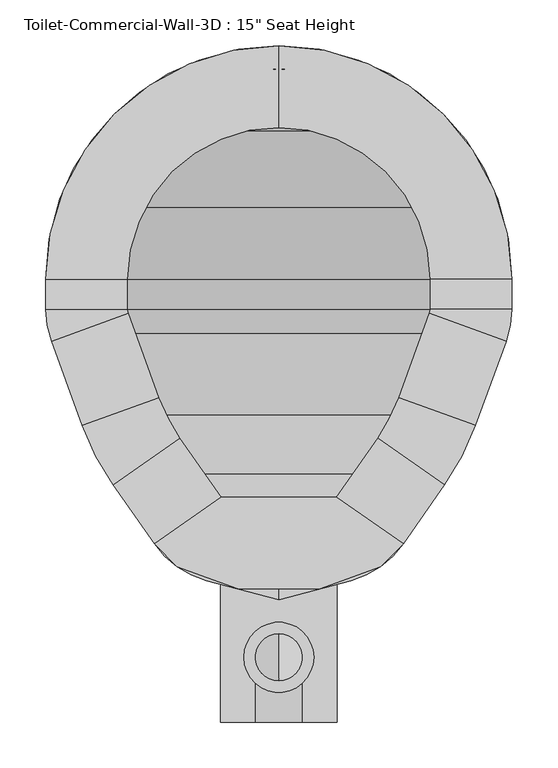
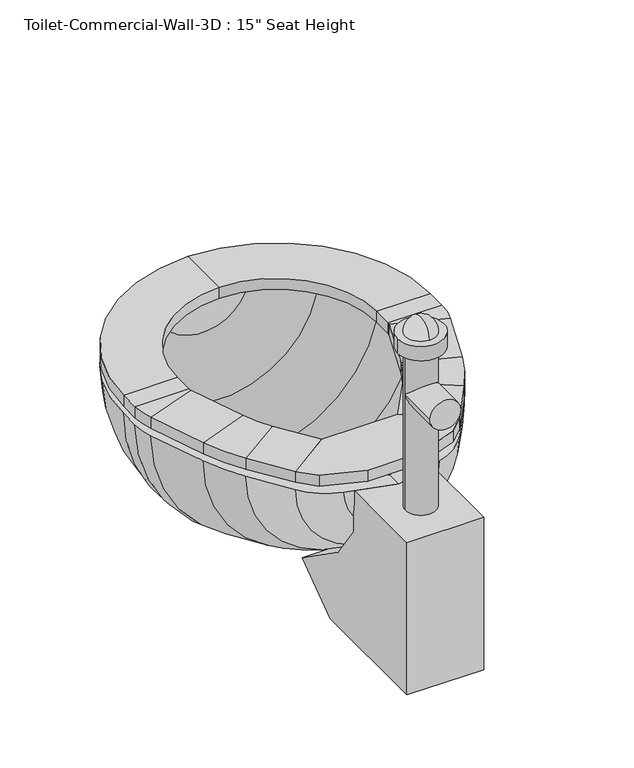
"""IFC4 building model written with IfcOpenShell, lengths in millimetres: flow terminal geometry."""

import ifcopenshell
import ifcopenshell.guid

model = None  # the IFC model being written
_history = None  # IfcOwnerHistory: only IFC2X3 demands one
_inside = {}  # id of a spatial element -> (the spatial element, [elements in it])
_under = {}  # id of a project, library or spatial element -> (it, [spatial elements below it])
_declared = {}  # id of a project -> (the project, [libraries it declares])
_typed = {}  # id of a type object -> (the type object, [elements of that type])
_made_of = {}  # id of a material, layer set ... -> (it, [elements and type objects made of it])


def new_model(schema):
    """Start an empty IFC model of exactly this schema.

    Asked for "IFC4X3", IfcOpenShell would pick the latest addendum, in which some entities
    have other attributes; the version numbers below select the first issue.
    IFC2X3 requires an IfcOwnerHistory on every rooted entity: one is made here for all.
    """
    global model, _history
    if schema == "IFC4X3":
        model = ifcopenshell.file(schema_version=(4, 3, 0, 0))
    else:
        model = ifcopenshell.file(schema=schema)
    _inside.clear()
    _under.clear()
    _declared.clear()
    _typed.clear()
    _made_of.clear()
    _history = None
    if model.schema == "IFC2X3":
        org = make("IfcOrganization", Name="unknown")
        user = make(
            "IfcPersonAndOrganization",
            ThePerson=make("IfcPerson", FamilyName="unknown"),
            TheOrganization=org,
        )
        app = make(
            "IfcApplication",
            ApplicationDeveloper=org,
            Version="unknown",
            ApplicationFullName="unknown",
            ApplicationIdentifier="unknown",
        )
        _history = make(
            "IfcOwnerHistory",
            OwningUser=user,
            OwningApplication=app,
            ChangeAction="ADDED",
            CreationDate=0,
        )
    return model


def make(cls, **values):
    """One entity of the class cls with the attributes given. An attribute that is None is left unset."""
    return model.create_entity(
        cls, **{name: value for name, value in values.items() if value is not None}
    )


def rooted(cls, **values):
    """An entity with a GlobalId (a new one), such as an element, a storey or a relation."""
    return make(cls, GlobalId=ifcopenshell.guid.new(), OwnerHistory=_history, **values)


def si_unit(unit_type, name, prefix=None):
    """IfcSIUnit, for example si_unit("LENGTHUNIT", "METRE", prefix="MILLI")."""
    return make("IfcSIUnit", UnitType=unit_type, Prefix=prefix, Name=name)


def assignment(units):
    """IfcUnitAssignment: the units of a project."""
    return None if units is None else make("IfcUnitAssignment", Units=units)


def point(xyz):
    """IfcCartesianPoint."""
    return None if xyz is None else make("IfcCartesianPoint", Coordinates=xyz)


def direction(xyz):
    """IfcDirection."""
    return None if xyz is None else make("IfcDirection", DirectionRatios=xyz)


def frame(location, z_axis=None, x_axis=None):
    """IfcAxis2Placement3D, a coordinate frame: its origin and axes. An axis left out is left unset."""
    return make(
        "IfcAxis2Placement3D",
        Location=point(location),
        Axis=direction(z_axis),
        RefDirection=direction(x_axis),
    )


def frame_2d(location, x_axis=None):
    """IfcAxis2Placement2D, a coordinate frame in the plane: its origin and x axis."""
    return make(
        "IfcAxis2Placement2D", Location=point(location), RefDirection=direction(x_axis)
    )


def origin():
    """The frame at (0, 0, 0) with its axes left unset."""
    return frame((0.0, 0.0, 0.0))


def place(relative_to, where):
    """IfcLocalPlacement: puts the frame where relative to a parent placement (None: the world)."""
    return make(
        "IfcLocalPlacement", PlacementRelTo=relative_to, RelativePlacement=where
    )


def context(
    kind, dimensions, precision=None, world=None, true_north=None, identifier=None
):
    """IfcGeometricRepresentationContext, for example the 3D "Model" context."""
    return make(
        "IfcGeometricRepresentationContext",
        ContextIdentifier=identifier,
        ContextType=kind,
        CoordinateSpaceDimension=dimensions,
        Precision=precision,
        WorldCoordinateSystem=world,
        TrueNorth=true_north,
    )


def project(units=None, contexts=None):
    """IfcProject with its units and contexts."""
    return rooted(
        "IfcProject",
        Name="project",
        RepresentationContexts=contexts,
        UnitsInContext=assignment(units),
    )


def spatial(cls, under=None, at=None, **own):
    """A site, building, storey or space (cls), placed at a placement, below another one or the project."""
    s = rooted(cls, ObjectPlacement=at, **own)
    if under is not None:
        _under.setdefault(under.id(), (under, []))[1].append(s)
    return s


def polyline(points):
    """IfcPolyline through the points."""
    return make("IfcPolyline", Points=[point(p) for p in points])


def circle_curve(where, radius):
    """IfcCircle in the frame where."""
    return make("IfcCircle", Position=where, Radius=radius)


def ellipse_curve(where, semi_axis1, semi_axis2):
    """IfcEllipse in the frame where."""
    return make(
        "IfcEllipse", Position=where, SemiAxis1=semi_axis1, SemiAxis2=semi_axis2
    )


def trimmed(basis, trim1, trim2, sense, master):
    """IfcTrimmedCurve: the piece of a basis curve between two trims."""
    return make(
        "IfcTrimmedCurve",
        BasisCurve=basis,
        Trim1=trim1,
        Trim2=trim2,
        SenseAgreement=sense,
        MasterRepresentation=master,
    )


def segment(curve, same_sense, transition):
    """IfcCompositeCurveSegment."""
    return make(
        "IfcCompositeCurveSegment",
        Transition=transition,
        SameSense=same_sense,
        ParentCurve=curve,
    )


def composite_curve(segments, self_intersect=None):
    """IfcCompositeCurve: segments joined end to end."""
    return make("IfcCompositeCurve", Segments=segments, SelfIntersect=self_intersect)


def outline(outer, holes=None, kind="AREA"):
    """IfcArbitraryClosedProfileDef: a profile drawn as a closed curve; with holes, ...WithVoids."""
    if holes is None:
        return make("IfcArbitraryClosedProfileDef", ProfileType=kind, OuterCurve=outer)
    return make(
        "IfcArbitraryProfileDefWithVoids",
        ProfileType=kind,
        OuterCurve=outer,
        InnerCurves=holes,
    )


def extrude(swept, where, along, depth):
    """IfcExtrudedAreaSolid: the profile swept, set in the frame where, extruded along a direction by depth."""
    return make(
        "IfcExtrudedAreaSolid",
        SweptArea=swept,
        Position=where,
        ExtrudedDirection=direction(along),
        Depth=depth,
    )


def shape(context_of_items, identifier, shape_type, items):
    """IfcShapeRepresentation: the items that make up one representation, for example the "Body"."""
    return make(
        "IfcShapeRepresentation",
        ContextOfItems=context_of_items,
        RepresentationIdentifier=identifier,
        RepresentationType=shape_type,
        Items=items,
    )


def source(mapping_origin, context_of_items, identifier, shape_type, items):
    """IfcRepresentationMap: a shape defined once, which mapped items show again and again."""
    return make(
        "IfcRepresentationMap",
        MappingOrigin=mapping_origin,
        MappedRepresentation=shape(context_of_items, identifier, shape_type, items),
    )


def transform(
    local_origin,
    x_axis=None,
    y_axis=None,
    z_axis=None,
    scale=None,
    scale2=None,
    scale3=None,
    uniform=True,
):
    """IfcCartesianTransformationOperator3D, or its non-uniform kind. x_axis, y_axis, z_axis: its Axis1, 2, 3."""
    if uniform:
        return make(
            "IfcCartesianTransformationOperator3D",
            Axis1=direction(x_axis),
            Axis2=direction(y_axis),
            LocalOrigin=point(local_origin),
            Scale=scale,
            Axis3=direction(z_axis),
        )
    return make(
        "IfcCartesianTransformationOperator3DnonUniform",
        Axis1=direction(x_axis),
        Axis2=direction(y_axis),
        LocalOrigin=point(local_origin),
        Scale=scale,
        Axis3=direction(z_axis),
        Scale2=scale2,
        Scale3=scale3,
    )


def mapped(mapping_source, mapping_target):
    """IfcMappedItem: shows the shape of a source again, moved by a transform."""
    return make(
        "IfcMappedItem", MappingSource=mapping_source, MappingTarget=mapping_target
    )


def made_of(thing, what):
    """Note that an element or type object is made of a material, layer set ...; save() writes the relation."""
    if what is not None:
        _made_of.setdefault(what.id(), (what, []))[1].append(thing)
    return thing


def element(
    cls,
    number,
    at=None,
    inside=None,
    cuts=None,
    type_object=None,
    material=None,
    context=None,
    identifier="Body",
    shape_type=None,
    held_by="IfcProductDefinitionShape",
    body=None,
    shapes=None,
    **own,
):
    """One element of the class cls, such as IfcWall. Its Tag is "e" and its number.

    at: its placement. inside: the storey or other place that contains it. cuts: it is an
    opening in that element (IfcRelVoidsElement). A single representation is given by context,
    identifier, shape_type and body (its items); several are given by shapes. held_by: the class
    of the entity that holds the representations. save() writes the other relations.
    """
    e = rooted(cls, Tag="e%d" % number, ObjectPlacement=at, **own)
    if body is not None:
        shapes = [shape(context, identifier, shape_type, body)]
    if shapes is not None:
        e.Representation = make(held_by, Representations=shapes)
    if inside is not None:
        _inside.setdefault(inside.id(), (inside, []))[1].append(e)
    if cuts is not None:
        rooted(
            "IfcRelVoidsElement", RelatingBuildingElement=cuts, RelatedOpeningElement=e
        )
    if type_object is not None:
        _typed.setdefault(type_object.id(), (type_object, []))[1].append(e)
    return made_of(e, material)


def aggregate(whole, parts):
    """IfcRelAggregates: a whole, such as a stair, and the parts it consists of."""
    return rooted("IfcRelAggregates", RelatingObject=whole, RelatedObjects=parts)


def save(model, path):
    """Write the relations noted so far, then the file.

    IfcRelAggregates (storeys below a building ...), IfcRelContainedInSpatialStructure (elements
    in a storey), IfcRelDefinesByType, IfcRelAssociatesMaterial and IfcRelDeclares: one each for
    every whole, place, type object, material and project.
    """
    for whole, parts in _under.values():
        aggregate(whole, parts)
    for where, things in _inside.values():
        rooted(
            "IfcRelContainedInSpatialStructure",
            RelatedElements=things,
            RelatingStructure=where,
        )
    for kind, things in _typed.values():
        rooted("IfcRelDefinesByType", RelatedObjects=things, RelatingType=kind)
    for what, things in _made_of.values():
        rooted("IfcRelAssociatesMaterial", RelatedObjects=things, RelatingMaterial=what)
    for by, libraries in _declared.values():
        rooted("IfcRelDeclares", RelatingContext=by, RelatedDefinitions=libraries)
    model.write(path)


def plane_surface(at):
    """IfcPlane: the flat surface through the origin of the frame at, square to its z axis."""
    return make("IfcPlane", Position=at)


def cylinder_surface(at, radius):
    """IfcCylindricalSurface: all points at the distance radius from the z axis of the frame at."""
    return make("IfcCylindricalSurface", Position=at, Radius=radius)


def revolved_surface(curve, axis_point, axis_direction):
    """IfcSurfaceOfRevolution: the curve turned about the line through axis_point along axis_direction."""
    return make(
        "IfcSurfaceOfRevolution",
        SweptCurve=make("IfcArbitraryOpenProfileDef", ProfileType="CURVE", Curve=curve),
        AxisPosition=make("IfcAxis1Placement", Location=point(axis_point), Axis=direction(axis_direction)),
    )


def advanced_brep(points, edges, surfaces, faces):
    """IfcAdvancedBrep: a solid bounded by faces that lie on surfaces and meet in shared edges.

    An edge is (start, end): straight between two places in points (the first is 0);
    or (start, end, curve); or (start, end, curve, False) where it runs against its curve.
    A face is (place in surfaces, loops), or (place, loops, False) where it looks against
    its surface's normal. A loop lists edges by number (the first is 1), with a minus sign
    where the edge is run from its end to its start. The first loop is the outer one.
    """
    corners = [point(p) for p in points]
    vertices = [make("IfcVertexPoint", VertexGeometry=c) for c in corners]
    made = []
    for start, end, *more in edges:
        made.append(
            make(
                "IfcEdgeCurve",
                EdgeStart=vertices[start],
                EdgeEnd=vertices[end],
                EdgeGeometry=more[0] if more else make("IfcPolyline", Points=[corners[start], corners[end]]),
                SameSense=more[1] if len(more) > 1 else True,
            )
        )
    hull = []
    for where, loops, *sense in faces:
        bounds = []
        for j, loop in enumerate(loops):
            ring = [make("IfcOrientedEdge", EdgeElement=made[abs(k) - 1], Orientation=k > 0) for k in loop]
            bounds.append(
                make(
                    "IfcFaceOuterBound" if j == 0 else "IfcFaceBound",
                    Bound=make("IfcEdgeLoop", EdgeList=ring),
                    Orientation=True,
                )
            )
        hull.append(make("IfcAdvancedFace", Bounds=bounds, FaceSurface=surfaces[where], SameSense=sense[0] if sense else True))
    return make("IfcAdvancedBrep", Outer=make("IfcClosedShell", CfsFaces=hull))


def flow_terminal_fb6ce90a(model_context):
    return source(origin(), model_context, "Body", "SolidModel", [
        extrude(outline(polyline([(467.7541169, 443.4722495), (540.5767337, 392.4813043), (515.6262519, 367.5308226), (449.563909, 343.4860961), (360.2423986, 343.4860961), (294.1800557, 367.5308226), (269.229574, 392.4813043), (342.0521907, 443.4722495), (467.7541169, 443.4722495)])), frame((0.0, 0.0, 355.6), z_axis=(0.0, 0.0, 1.0), x_axis=(1.0, 0.0, 0.0)), (0.0, 0.0, 1.0), 19.05),
        advanced_brep(
        [(467.7541169, 443.4722495, 355.6), (540.5767337, 392.4813043, 355.6), (540.5767337, 392.4813043, 374.65), (467.7541169, 443.4722495, 374.65), (512.8583992, 507.8878403, 355.6), (585.6810159, 456.8968951, 355.6), (585.6810159, 456.8968951, 374.65), (512.8583992, 507.8878403, 374.65), (619.360053, 521.5937234, 355.6), (535.821379, 551.9993141, 355.6), (619.360053, 521.5937234, 374.65), (535.821379, 551.9993141, 374.65), (569.2372501, 643.8086654, 355.6), (652.7759241, 613.4030747, 355.6), (652.7759241, 613.4030747, 374.65), (569.2372501, 643.8086654, 374.65), (658.9031538, 648.1523212, 355.6), (570.0031538, 648.1523212, 355.6), (658.9031538, 648.1523212, 374.65), (570.0031538, 648.1523212, 374.65), (570.0031538, 681.0375, 355.6), (658.9031538, 681.0375, 355.6), (658.9031538, 681.0375, 374.65), (570.0031538, 681.0375, 374.65), (404.9031538, 935.0375, 355.6), (404.9031538, 846.1375, 355.6), (404.9031538, 935.0375, 374.65), (404.9031538, 846.1375, 374.65), (150.9031538, 681.0375, 355.6), (239.8031538, 681.0375, 355.6), (150.9031538, 681.0375, 374.65), (239.8031538, 681.0375, 374.65), (239.8031538, 648.1523212, 355.6), (150.9031538, 648.1523212, 355.6), (150.9031538, 648.1523212, 374.65), (239.8031538, 648.1523212, 374.65), (157.0303835, 613.4030747, 355.6), (240.5690575, 643.8086654, 355.6), (157.0303835, 613.4030747, 374.65), (240.5690575, 643.8086654, 374.65), (273.9849286, 551.9993141, 355.6), (190.4462546, 521.5937234, 355.6), (190.4462546, 521.5937234, 374.65), (273.9849286, 551.9993141, 374.65), (224.1252917, 456.8968951, 355.6), (296.9479084, 507.8878403, 355.6), (224.1252917, 456.8968951, 374.65), (296.9479084, 507.8878403, 374.65), (342.0521907, 443.4722495, 355.6), (342.0521907, 443.4722495, 374.65), (269.229574, 392.4813043, 374.65), (269.229574, 392.4813043, 355.6)],
        [
            (0, 1),
            (1, 2),
            (2, 3),
            (3, 0),
            (0, 4),
            (4, 5),
            (5, 1),
            (5, 6),
            (6, 2),
            (6, 7),
            (7, 3),
            (7, 4),
            (8, 5, circle_curve(frame((356.8099347, 617.1541514, 355.6), z_axis=(0.0, 0.0, -1.0), x_axis=(0.81915204428899, -0.5735764363510486, 0.0)), 279.4)),
            (4, 9, circle_curve(frame((356.8099347, 617.1541514, 355.6), z_axis=(0.0, 0.0, 1.0), x_axis=(0.81915204428899, -0.5735764363510486, 0.0)), 190.5)),
            (9, 8),
            (10, 6, circle_curve(frame((356.8099347, 617.1541514, 374.65), z_axis=(0.0, 0.0, -1.0), x_axis=(0.81915204428899, -0.5735764363510486, 0.0)), 279.4)),
            (8, 10),
            (11, 7, circle_curve(frame((356.8099347, 617.1541514, 374.65), z_axis=(0.0, 0.0, -1.0), x_axis=(0.81915204428899, -0.5735764363510486, 0.0)), 190.5)),
            (10, 11),
            (11, 9),
            (9, 12),
            (12, 13),
            (13, 8),
            (13, 14),
            (14, 10),
            (14, 15),
            (15, 11),
            (15, 12),
            (16, 13, circle_curve(frame((557.3031538, 648.1523212, 355.6), z_axis=(0.0, 0.0, -1.0), x_axis=(0.9396926207859057, -0.3420201433256761, 0.0)), 101.6)),
            (12, 17, circle_curve(frame((557.3031538, 648.1523212, 355.6), z_axis=(0.0, 0.0, 1.0), x_axis=(0.9396926207859057, -0.3420201433256761, 0.0)), 12.7)),
            (17, 16),
            (18, 14, circle_curve(frame((557.3031538, 648.1523212, 374.65), z_axis=(0.0, 0.0, -1.0), x_axis=(0.9396926207859057, -0.3420201433256761, 0.0)), 101.6)),
            (16, 18),
            (19, 15, circle_curve(frame((557.3031538, 648.1523212, 374.65), z_axis=(0.0, 0.0, -1.0), x_axis=(0.9396926207859057, -0.3420201433256761, 0.0)), 12.7)),
            (18, 19),
            (19, 17),
            (17, 20),
            (20, 21),
            (21, 16),
            (21, 22),
            (22, 18),
            (22, 23),
            (23, 19),
            (23, 20),
            (24, 21, circle_curve(frame((404.9031538, 681.0375, 355.6), z_axis=(0.0, 0.0, -1.0), x_axis=(1.0, 0.0, 0.0)), 254.0)),
            (20, 25, circle_curve(frame((404.9031538, 681.0375, 355.6), z_axis=(0.0, 0.0, 1.0), x_axis=(1.0, 0.0, 0.0)), 165.1)),
            (25, 24),
            (26, 22, circle_curve(frame((404.9031538, 681.0375, 374.65), z_axis=(0.0, 0.0, -1.0), x_axis=(1.0, 0.0, 0.0)), 254.0)),
            (24, 26),
            (27, 23, circle_curve(frame((404.9031538, 681.0375, 374.65), z_axis=(0.0, 0.0, -1.0), x_axis=(1.0, 0.0, 0.0)), 165.1)),
            (26, 27),
            (27, 25),
            (28, 24, circle_curve(frame((404.9031538, 681.0375, 355.6), z_axis=(0.0, 0.0, -1.0), x_axis=(0.0, 1.0, 0.0)), 254.0)),
            (25, 29, circle_curve(frame((404.9031538, 681.0375, 355.6), z_axis=(0.0, 0.0, 1.0), x_axis=(0.0, 1.0, 0.0)), 165.1)),
            (29, 28),
            (30, 26, circle_curve(frame((404.9031538, 681.0375, 374.65), z_axis=(0.0, 0.0, -1.0), x_axis=(0.0, 1.0, 0.0)), 254.0)),
            (28, 30),
            (31, 27, circle_curve(frame((404.9031538, 681.0375, 374.65), z_axis=(0.0, 0.0, -1.0), x_axis=(0.0, 1.0, 0.0)), 165.1)),
            (30, 31),
            (31, 29),
            (29, 32),
            (32, 33),
            (33, 28),
            (33, 34),
            (34, 30),
            (34, 35),
            (35, 31),
            (35, 32),
            (36, 33, circle_curve(frame((252.5031538, 648.1523212, 355.6), z_axis=(0.0, 0.0, -1.0), x_axis=(-1.0, 0.0, 0.0)), 101.6)),
            (32, 37, circle_curve(frame((252.5031538, 648.1523212, 355.6), z_axis=(0.0, 0.0, 1.0), x_axis=(-1.0, 0.0, 0.0)), 12.7)),
            (37, 36),
            (38, 34, circle_curve(frame((252.5031538, 648.1523212, 374.65), z_axis=(0.0, 0.0, -1.0), x_axis=(-1.0, 0.0, 0.0)), 101.6)),
            (36, 38),
            (39, 35, circle_curve(frame((252.5031538, 648.1523212, 374.65), z_axis=(0.0, 0.0, -1.0), x_axis=(-1.0, 0.0, 0.0)), 12.7)),
            (38, 39),
            (39, 37),
            (37, 40),
            (40, 41),
            (41, 36),
            (41, 42),
            (42, 38),
            (42, 43),
            (43, 39),
            (43, 40),
            (44, 41, circle_curve(frame((452.9963729, 617.1541514, 355.6), z_axis=(0.0, 0.0, -1.0), x_axis=(-0.939692620785909, -0.3420201433256672, 0.0)), 279.4)),
            (40, 45, circle_curve(frame((452.9963729, 617.1541514, 355.6), z_axis=(0.0, 0.0, 1.0), x_axis=(-0.939692620785909, -0.3420201433256672, 0.0)), 190.5)),
            (45, 44),
            (46, 42, circle_curve(frame((452.9963729, 617.1541514, 374.65), z_axis=(0.0, 0.0, -1.0), x_axis=(-0.939692620785909, -0.3420201433256672, 0.0)), 279.4)),
            (44, 46),
            (47, 43, circle_curve(frame((452.9963729, 617.1541514, 374.65), z_axis=(0.0, 0.0, -1.0), x_axis=(-0.939692620785909, -0.3420201433256672, 0.0)), 190.5)),
            (46, 47),
            (47, 45),
            (48, 49),
            (49, 50),
            (50, 51),
            (51, 48),
            (45, 48),
            (51, 44),
            (50, 46),
            (49, 47),
        ],
        [
            plane_surface(frame((540.5767337, 392.4813043, 437.2995365), z_axis=(-0.5735764363510436, -0.8191520442889937, 0.0), x_axis=(0.8191520442889937, -0.5735764363510436, 0.0))),
            plane_surface(frame((467.7541169, 443.4722495, 355.6), z_axis=(0.0, 0.0, -1.0), x_axis=(0.5735764363510436, 0.8191520442889936, 0.0))),
            plane_surface(frame((540.5767337, 392.4813043, 355.6), z_axis=(0.8191520442889944, -0.5735764363510424, 0.0), x_axis=(0.5735764363510424, 0.8191520442889944, 0.0))),
            plane_surface(frame((540.5767337, 392.4813043, 374.65), z_axis=(0.0, 0.0, 1.0), x_axis=(0.573576436351043, 0.819152044288994, 0.0))),
            plane_surface(frame((467.7541169, 443.4722495, 374.65), z_axis=(-0.819152044288994, 0.573576436351043, 0.0), x_axis=(0.573576436351043, 0.819152044288994, 0.0))),
            plane_surface(frame((356.8099347, 617.1541514, 355.6), z_axis=(0.0, 0.0, -1.0), x_axis=(0.81915204428899, -0.5735764363510486, 0.0))),
            cylinder_surface(frame((356.8099347, 617.1541514, 342.9), z_axis=(0.0, 0.0, 1.0), x_axis=(0.81915204428899, -0.5735764363510486, 0.0)), 279.4),
            plane_surface(frame((356.8099347, 617.1541514, 374.65), z_axis=(0.0, 0.0, 1.0), x_axis=(0.81915204428899, -0.5735764363510486, 0.0))),
            revolved_surface(polyline([(512.8583991370526, 507.8878402751253, 374.65), (512.8583991370526, 507.8878402751253, 355.6)]), (356.8099347, 617.1541514, 342.9), (0.0, 0.0, 1.0)),
            plane_surface(frame((535.821379, 551.9993141, 355.6), z_axis=(0.0, 0.0, -1.0000000000000002), x_axis=(0.3420201433256594, 0.9396926207859119, 0.0))),
            plane_surface(frame((619.360053, 521.5937234, 355.6), z_axis=(0.9396926207859121, -0.3420201433256587, 0.0), x_axis=(0.3420201433256587, 0.9396926207859121, 0.0))),
            plane_surface(frame((619.360053, 521.5937234, 374.65), z_axis=(0.0, 0.0, 1.0), x_axis=(0.34202014332565916, 0.9396926207859119, 0.0))),
            plane_surface(frame((535.821379, 551.9993141, 374.65), z_axis=(-0.9396926207859122, 0.34202014332565833, 0.0), x_axis=(0.34202014332565833, 0.9396926207859122, 0.0))),
            plane_surface(frame((557.3031538, 648.1523212, 355.6), z_axis=(0.0, 0.0, -1.0000000000000002), x_axis=(0.9396926207859058, -0.34202014332567615, 0.0))),
            cylinder_surface(frame((557.3031538, 648.1523212, 342.9), z_axis=(0.0, 0.0, 1.0), x_axis=(0.9396926207859057, -0.3420201433256761, 0.0)), 101.6),
            plane_surface(frame((557.3031538, 648.1523212, 374.65), z_axis=(0.0, 0.0, 1.0000000000000002), x_axis=(0.9396926207859058, -0.34202014332567615, 0.0))),
            revolved_surface(polyline([(569.237250083981, 643.8086653797639, 374.65), (569.237250083981, 643.8086653797639, 355.6)]), (557.3031538, 648.1523212, 342.9), (0.0, 0.0, 1.0)),
            plane_surface(frame((570.0031538, 648.1523212, 355.6), z_axis=(0.0, 0.0, -1.0), x_axis=(0.0, 1.0, 0.0))),
            plane_surface(frame((658.9031538, 648.1523212, 355.6), z_axis=(1.0, 0.0, 0.0), x_axis=(0.0, 1.0, 0.0))),
            plane_surface(frame((658.9031538, 648.1523212, 374.65), z_axis=(0.0, 0.0, 1.0), x_axis=(0.0, 1.0, 0.0))),
            plane_surface(frame((570.0031538, 648.1523212, 374.65), z_axis=(-1.0, 0.0, 0.0), x_axis=(0.0, 1.0, 0.0))),
            plane_surface(frame((404.9031538, 681.0375, 355.6), z_axis=(0.0, 0.0, -1.0), x_axis=(1.0, 0.0, 0.0))),
            cylinder_surface(frame((404.9031538, 681.0375, 342.9), z_axis=(0.0, 0.0, 1.0), x_axis=(1.0, 0.0, 0.0)), 254.0),
            plane_surface(frame((404.9031538, 681.0375, 374.65), z_axis=(0.0, 0.0, 1.0), x_axis=(1.0, 0.0, 0.0))),
            revolved_surface(polyline([(570.0031538, 681.0375, 374.65), (570.0031538, 681.0375, 355.6)]), (404.9031538, 681.0375, 342.9), (0.0, 0.0, 1.0)),
            plane_surface(frame((404.9031538, 681.0375, 355.6), z_axis=(0.0, 0.0, -1.0), x_axis=(0.0, 1.0, 0.0))),
            cylinder_surface(frame((404.9031538, 681.0375, 342.9), z_axis=(0.0, 0.0, 1.0), x_axis=(0.0, 1.0, 0.0)), 254.0),
            plane_surface(frame((404.9031538, 681.0375, 374.65), z_axis=(0.0, 0.0, 1.0), x_axis=(0.0, 1.0, 0.0))),
            revolved_surface(polyline([(404.9031538, 846.1375, 374.65), (404.9031538, 846.1375, 355.6)]), (404.9031538, 681.0375, 342.9), (0.0, 0.0, 1.0)),
            plane_surface(frame((239.8031538, 681.0375, 355.6), z_axis=(0.0, 0.0, -1.0), x_axis=(0.0, -1.0, 0.0))),
            plane_surface(frame((150.9031538, 681.0375, 355.6), z_axis=(-1.0, 0.0, 0.0), x_axis=(0.0, -1.0, 0.0))),
            plane_surface(frame((150.9031538, 681.0375, 374.65), z_axis=(0.0, 0.0, 1.0), x_axis=(0.0, -1.0, 0.0))),
            plane_surface(frame((239.8031538, 681.0375, 374.65), z_axis=(1.0, 0.0, 0.0), x_axis=(0.0, -1.0, 0.0))),
            plane_surface(frame((252.5031538, 648.1523212, 355.6), z_axis=(0.0, 0.0, -1.0), x_axis=(-1.0, 0.0, 0.0))),
            cylinder_surface(frame((252.5031538, 648.1523212, 342.9), z_axis=(0.0, 0.0, 1.0), x_axis=(-1.0, 0.0, 0.0)), 101.6),
            plane_surface(frame((252.5031538, 648.1523212, 374.65), z_axis=(0.0, 0.0, 1.0), x_axis=(-1.0, 0.0, 0.0))),
            revolved_surface(polyline([(239.80315380000002, 648.1523212, 374.65), (239.80315380000002, 648.1523212, 355.6)]), (252.5031538, 648.1523212, 342.9), (0.0, 0.0, 1.0)),
            plane_surface(frame((240.5690575, 643.8086654, 355.6), z_axis=(0.0, 0.0, -1.0), x_axis=(0.3420201433256581, -0.9396926207859123, 0.0))),
            plane_surface(frame((157.0303835, 613.4030747, 355.6), z_axis=(-0.9396926207859122, -0.3420201433256583, 0.0), x_axis=(0.3420201433256583, -0.9396926207859122, 0.0))),
            plane_surface(frame((157.0303835, 613.4030747, 374.65), z_axis=(0.0, 0.0, 1.0), x_axis=(0.34202014332565855, -0.9396926207859121, 0.0))),
            plane_surface(frame((240.5690575, 643.8086654, 374.65), z_axis=(0.9396926207859124, 0.3420201433256579, 0.0), x_axis=(0.3420201433256579, -0.9396926207859124, 0.0))),
            plane_surface(frame((452.9963729, 617.1541514, 355.6), z_axis=(0.0, 0.0, -1.0), x_axis=(-0.939692620785909, -0.3420201433256672, 0.0))),
            cylinder_surface(frame((452.9963729, 617.1541514, 342.9), z_axis=(0.0, 0.0, 1.0), x_axis=(-0.939692620785909, -0.3420201433256672, 0.0)), 279.4),
            plane_surface(frame((452.9963729, 617.1541514, 374.65), z_axis=(0.0, 0.0, 1.0), x_axis=(-0.939692620785909, -0.3420201433256672, 0.0))),
            revolved_surface(polyline([(273.98492864028435, 551.9993140964605, 374.65), (273.98492864028435, 551.9993140964605, 355.6)]), (452.9963729, 617.1541514, 342.9), (0.0, 0.0, 1.0)),
            plane_surface(frame((269.229574, 392.4813043, 248.5004635), z_axis=(0.5735764363510469, -0.8191520442889914, 0.0), x_axis=(0.8191520442889914, 0.5735764363510469, 0.0))),
            plane_surface(frame((296.9479084, 507.8878403, 355.6), z_axis=(0.0, 0.0, -1.0), x_axis=(0.5735764363510465, -0.8191520442889916, 0.0))),
            plane_surface(frame((224.1252917, 456.8968951, 355.6), z_axis=(-0.819152044288991, -0.5735764363510473, 0.0), x_axis=(0.5735764363510473, -0.819152044288991, 0.0))),
            plane_surface(frame((224.1252917, 456.8968951, 374.65), z_axis=(0.0, 0.0, 1.0), x_axis=(0.5735764363510473, -0.819152044288991, 0.0))),
            plane_surface(frame((296.9479084, 507.8878403, 374.65), z_axis=(0.8191520442889914, 0.5735764363510468, 0.0), x_axis=(0.5735764363510468, -0.8191520442889914, 0.0))),
        ],
        [
            (0, [[1, 2, 3, 4]]),
            (1, [[-1, 5, 6, 7]]),
            (2, [[-2, -7, 8, 9]]),
            (3, [[-3, -9, 10, 11]]),
            (4, [[-4, -11, 12, -5]]),
            (5, [[13, -6, 14, 15]]),
            (6, [[16, -8, -13, 17]]),
            (7, [[18, -10, -16, 19]]),
            (8, [[-14, -12, -18, 20]]),
            (9, [[-15, 21, 22, 23]]),
            (10, [[-17, -23, 24, 25]]),
            (11, [[-19, -25, 26, 27]]),
            (12, [[-20, -27, 28, -21]]),
            (13, [[29, -22, 30, 31]]),
            (14, [[32, -24, -29, 33]]),
            (15, [[34, -26, -32, 35]]),
            (16, [[-30, -28, -34, 36]]),
            (17, [[-31, 37, 38, 39]]),
            (18, [[-33, -39, 40, 41]]),
            (19, [[-35, -41, 42, 43]]),
            (20, [[-36, -43, 44, -37]]),
            (21, [[45, -38, 46, 47]]),
            (22, [[48, -40, -45, 49]]),
            (23, [[50, -42, -48, 51]]),
            (24, [[-46, -44, -50, 52]]),
            (25, [[53, -47, 54, 55]]),
            (26, [[56, -49, -53, 57]]),
            (27, [[58, -51, -56, 59]]),
            (28, [[-54, -52, -58, 60]]),
            (29, [[-55, 61, 62, 63]]),
            (30, [[-57, -63, 64, 65]]),
            (31, [[-59, -65, 66, 67]]),
            (32, [[-60, -67, 68, -61]]),
            (33, [[69, -62, 70, 71]]),
            (34, [[72, -64, -69, 73]]),
            (35, [[74, -66, -72, 75]]),
            (36, [[-70, -68, -74, 76]]),
            (37, [[-71, 77, 78, 79]]),
            (38, [[-73, -79, 80, 81]]),
            (39, [[-75, -81, 82, 83]]),
            (40, [[-76, -83, 84, -77]]),
            (41, [[85, -78, 86, 87]]),
            (42, [[88, -80, -85, 89]]),
            (43, [[90, -82, -88, 91]]),
            (44, [[-86, -84, -90, 92]]),
            (45, [[93, 94, 95, 96]]),
            (46, [[-87, 97, -96, 98]]),
            (47, [[-89, -98, -95, 99]]),
            (48, [[-91, -99, -94, 100]]),
            (49, [[-92, -100, -93, -97]]),
        ],
    ),
        advanced_brep(
        [(491.7762702, 919.7194257, 342.9), (404.9031538, 935.0375, 342.9), (404.9031538, 909.6375, 342.9), (483.0889586, 895.8512331, 342.9), (566.547764, 842.6821102, 342.9), (619.7168869, 759.2233048, 342.9), (633.5031538, 681.0375, 342.9), (633.5031538, 648.1523212, 342.9), (628.9077315, 622.0903863, 342.9), (596.6355667, 533.4233422, 342.9), (562.9565296, 468.7265139, 342.9), (525.0728964, 414.6230786, 342.9), (468.1430637, 374.7603806, 342.9), (404.9031538, 357.8152978, 342.9), (404.9031538, 331.5192829, 342.9), (483.6469009, 352.6186063, 342.9), (540.5767337, 392.4813043, 342.9), (585.6810159, 456.8968951, 342.9), (619.360053, 521.5937234, 342.9), (652.7759241, 613.4030747, 342.9), (658.9031538, 648.1523212, 342.9), (658.9031538, 681.0375, 342.9), (643.5850795, 767.9106164, 342.9), (584.5082762, 860.6426224, 342.9), (318.0300374, 919.7194257, 342.9), (225.2980314, 860.6426224, 342.9), (166.2212281, 767.9106164, 342.9), (150.9031538, 681.0375, 342.9), (150.9031538, 648.1523212, 342.9), (157.0303835, 613.4030747, 342.9), (190.4462546, 521.5937234, 342.9), (224.1252917, 456.8968951, 342.9), (269.229574, 392.4813043, 342.9), (326.1594067, 352.6186063, 342.9), (341.663244, 374.7603806, 342.9), (284.7334112, 414.6230786, 342.9), (246.849778, 468.7265139, 342.9), (213.1707409, 533.4233422, 342.9), (180.8985761, 622.0903863, 342.9), (176.3031538, 648.1523212, 342.9), (176.3031538, 681.0375, 342.9), (190.0894207, 759.2233048, 342.9), (243.2585436, 842.6821102, 342.9), (326.7173491, 895.8512331, 342.9)],
        [
            (0, 1, circle_curve(frame((404.9031538, 681.0375, 342.9), z_axis=(0.0, 0.0, 1.0), x_axis=(1.0, 0.0, 0.0)), 254.0)),
            (1, 2),
            (2, 3, circle_curve(frame((404.9031538, 681.0375, 342.9), z_axis=(0.0, 0.0, -1.0), x_axis=(1.0, 0.0, 0.0)), 228.6)),
            (3, 4, circle_curve(frame((404.9031538, 681.0375, 342.9), z_axis=(0.0, 0.0, -1.0), x_axis=(1.0, 0.0, 0.0)), 228.6)),
            (4, 5, circle_curve(frame((404.9031538, 681.0375, 342.9), z_axis=(0.0, 0.0, -1.0), x_axis=(1.0, 0.0, 0.0)), 228.6)),
            (5, 6, circle_curve(frame((404.9031538, 681.0375, 342.9), z_axis=(0.0, 0.0, -1.0), x_axis=(1.0, 0.0, 0.0)), 228.6)),
            (6, 7),
            (7, 8, circle_curve(frame((557.3031538, 648.1523212, 342.9), z_axis=(0.0, 0.0, -1.0), x_axis=(1.0, 0.0, 0.0)), 76.2)),
            (8, 9),
            (9, 10, circle_curve(frame((334.0854485, 628.9837703, 342.9), z_axis=(0.0, 0.0, -1.0), x_axis=(1.0, 0.0, 0.0)), 279.4)),
            (10, 11),
            (11, 12, circle_curve(frame((441.8470487, 472.8984446, 342.9), z_axis=(0.0, 0.0, -1.0), x_axis=(1.0, 0.0, 0.0)), 101.6)),
            (12, 13),
            (13, 14),
            (14, 15),
            (15, 16, circle_curve(frame((457.350886, 450.7566703, 342.9), z_axis=(0.0, 0.0, 1.0), x_axis=(1.0, 0.0, 0.0)), 101.6)),
            (16, 17),
            (17, 18, circle_curve(frame((356.8099347, 617.1541514, 342.9), z_axis=(0.0, 0.0, 1.0), x_axis=(1.0, 0.0, 0.0)), 279.4)),
            (18, 19),
            (19, 20, circle_curve(frame((557.3031538, 648.1523212, 342.9), z_axis=(0.0, 0.0, 1.0), x_axis=(1.0, 0.0, 0.0)), 101.6)),
            (20, 21),
            (21, 22, circle_curve(frame((404.9031538, 681.0375, 342.9), z_axis=(0.0, 0.0, 1.0), x_axis=(1.0, 0.0, 0.0)), 254.0)),
            (22, 23, circle_curve(frame((404.9031538, 681.0375, 342.9), z_axis=(0.0, 0.0, 1.0), x_axis=(1.0, 0.0, 0.0)), 254.0)),
            (23, 0, circle_curve(frame((404.9031538, 681.0375, 342.9), z_axis=(0.0, 0.0, 1.0), x_axis=(1.0, 0.0, 0.0)), 254.0)),
            (24, 25, circle_curve(frame((404.9031538, 681.0375, 342.9), z_axis=(0.0, 0.0, 1.0), x_axis=(-1.0, 0.0, 0.0)), 254.0)),
            (25, 26, circle_curve(frame((404.9031538, 681.0375, 342.9), z_axis=(0.0, 0.0, 1.0), x_axis=(-1.0, 0.0, 0.0)), 254.0)),
            (26, 27, circle_curve(frame((404.9031538, 681.0375, 342.9), z_axis=(0.0, 0.0, 1.0), x_axis=(-1.0, 0.0, 0.0)), 254.0)),
            (27, 28),
            (28, 29, circle_curve(frame((252.5031538, 648.1523212, 342.9), z_axis=(0.0, 0.0, 1.0), x_axis=(-1.0, 0.0, 0.0)), 101.6)),
            (29, 30),
            (30, 31, circle_curve(frame((452.9963729, 617.1541514, 342.9), z_axis=(0.0, 0.0, 1.0), x_axis=(-1.0, 0.0, 0.0)), 279.4)),
            (31, 32),
            (32, 33, circle_curve(frame((352.4554217, 450.7566703, 342.9), z_axis=(0.0, 0.0, 1.0), x_axis=(-1.0, 0.0, 0.0)), 101.6)),
            (33, 14),
            (13, 34),
            (34, 35, circle_curve(frame((367.9592589, 472.8984446, 342.9), z_axis=(0.0, 0.0, -1.0), x_axis=(-1.0, 0.0, 0.0)), 101.6)),
            (35, 36),
            (36, 37, circle_curve(frame((475.7208592, 628.9837703, 342.9), z_axis=(0.0, 0.0, -1.0), x_axis=(-1.0, 0.0, 0.0)), 279.4)),
            (37, 38),
            (38, 39, circle_curve(frame((252.5031538, 648.1523212, 342.9), z_axis=(0.0, 0.0, -1.0), x_axis=(-1.0, 0.0, 0.0)), 76.2)),
            (39, 40),
            (40, 41, circle_curve(frame((404.9031538, 681.0375, 342.9), z_axis=(0.0, 0.0, -1.0), x_axis=(-1.0, 0.0, 0.0)), 228.6)),
            (41, 42, circle_curve(frame((404.9031538, 681.0375, 342.9), z_axis=(0.0, 0.0, -1.0), x_axis=(-1.0, 0.0, 0.0)), 228.6)),
            (42, 43, circle_curve(frame((404.9031538, 681.0375, 342.9), z_axis=(0.0, 0.0, -1.0), x_axis=(-1.0, 0.0, 0.0)), 228.6)),
            (43, 2, circle_curve(frame((404.9031538, 681.0375, 342.9), z_axis=(0.0, 0.0, -1.0), x_axis=(-1.0, 0.0, 0.0)), 228.6)),
            (1, 24, circle_curve(frame((404.9031538, 681.0375, 342.9), z_axis=(0.0, 0.0, 1.0), x_axis=(-1.0, 0.0, 0.0)), 254.0)),
            (0, 24, circle_curve(frame((404.9031538, 919.7194257, 342.9), z_axis=(0.0, 1.0, 0.0), x_axis=(1.0, 0.0, 0.0)), 86.8731164)),
            (43, 3, circle_curve(frame((404.9031538, 895.8512331, 342.9), z_axis=(0.0, -1.0, 0.0), x_axis=(1.0, 0.0, 0.0)), 78.1858048)),
            (42, 4, circle_curve(frame((404.9031538, 842.6821102, 342.9), z_axis=(0.0, -1.0, 0.0), x_axis=(1.0, 0.0, 0.0)), 161.6446102)),
            (41, 5, circle_curve(frame((404.9031538, 759.2233048, 342.9), z_axis=(0.0, -1.0, 0.0), x_axis=(1.0, 0.0, 0.0)), 214.8137331)),
            (40, 6, circle_curve(frame((404.9031538, 681.0375, 342.9), z_axis=(0.0, -1.0, 0.0), x_axis=(1.0, 0.0, 0.0)), 228.6)),
            (39, 7, circle_curve(frame((404.9031538, 648.1523212, 342.9), z_axis=(0.0, -1.0, 0.0), x_axis=(1.0, 0.0, 0.0)), 228.6)),
            (38, 8, circle_curve(frame((404.9031538, 622.0903863, 342.9), z_axis=(0.0, -1.0, 0.0), x_axis=(1.0, 0.0, 0.0)), 224.0045777)),
            (37, 9, circle_curve(frame((404.9031538, 533.4233422, 342.9), z_axis=(0.0, -1.0, 0.0), x_axis=(1.0, 0.0, 0.0)), 191.7324129)),
            (36, 10, circle_curve(frame((404.9031538, 468.7265139, 342.9), z_axis=(0.0, -1.0, 0.0), x_axis=(1.0, 0.0, 0.0)), 158.0533758)),
            (35, 11, circle_curve(frame((404.9031538, 414.6230786, 342.9), z_axis=(0.0, -1.0, 0.0), x_axis=(1.0, 0.0, 0.0)), 120.1697426)),
            (34, 12, circle_curve(frame((404.9031538, 374.7603806, 342.9), z_axis=(0.0, -1.0, 0.0), x_axis=(1.0, 0.0, 0.0)), 63.2399099)),
            (33, 15, circle_curve(frame((404.9031538, 352.6186063, 342.9), z_axis=(0.0, -1.0, 0.0), x_axis=(1.0, 0.0, 0.0)), 78.7437471)),
            (32, 16, circle_curve(frame((404.9031538, 392.4813043, 342.9), z_axis=(0.0, -1.0, 0.0), x_axis=(1.0, 0.0, 0.0)), 135.6735798)),
            (31, 17, circle_curve(frame((404.9031538, 456.8968951, 342.9), z_axis=(0.0, -1.0, 0.0), x_axis=(1.0, 0.0, 0.0)), 180.7778621)),
            (30, 18, circle_curve(frame((404.9031538, 521.5937234, 342.9), z_axis=(0.0, -1.0, 0.0), x_axis=(1.0, 0.0, 0.0)), 214.4568992)),
            (29, 19, circle_curve(frame((404.9031538, 613.4030747, 342.9), z_axis=(0.0, -1.0, 0.0), x_axis=(1.0, 0.0, 0.0)), 247.8727703)),
            (28, 20, circle_curve(frame((404.9031538, 648.1523212, 342.9), z_axis=(0.0, -1.0, 0.0), x_axis=(1.0, 0.0, 0.0)), 254.0)),
            (27, 21, circle_curve(frame((404.9031538, 681.0375, 342.9), z_axis=(0.0, -1.0, 0.0), x_axis=(1.0, 0.0, 0.0)), 254.0)),
            (26, 22, circle_curve(frame((404.9031538, 767.9106164, 342.9), z_axis=(0.0, -1.0, 0.0), x_axis=(1.0, 0.0, 0.0)), 238.6819257)),
            (25, 23, circle_curve(frame((404.9031538, 860.6426224, 342.9), z_axis=(0.0, -1.0, 0.0), x_axis=(1.0, 0.0, 0.0)), 179.6051224)),
        ],
        [
            plane_surface(frame((404.9031538, 1040.2477448, 342.9), z_axis=(0.0, 0.0, 1.0), x_axis=(1.0, 0.0, 0.0))),
            plane_surface(frame((404.9031538, 1040.2477448, 342.9), z_axis=(0.0, 0.0, 1.0), x_axis=(-1.0, 0.0, 0.0))),
            revolved_surface(trimmed(ellipse_curve(frame((404.9031538, 681.0375, 342.9), z_axis=(0.0, 0.0, 1.0), x_axis=(1.0, 0.0, 0.0)), 254.0, 254.0), [point((491.7762702, 919.7194257, 342.9))], [point((404.9031538, 935.0375, 342.9))], True, "CARTESIAN"), (404.9031538, 1040.2477448, 342.9), (0.0, 1.0, 0.0)),
            revolved_surface(trimmed(ellipse_curve(frame((404.9031538, 681.0375, 342.9), z_axis=(0.0, 0.0, -1.0), x_axis=(1.0, 0.0, 0.0)), 228.6, 228.6), [point((404.9031538, 909.6375, 342.9))], [point((483.0889586, 895.8512331, 342.9))], True, "CARTESIAN"), (404.9031538, 1040.2477448, 342.9), (0.0, 1.0, 0.0)),
            revolved_surface(trimmed(ellipse_curve(frame((404.9031538, 681.0375, 342.9), z_axis=(0.0, 0.0, -1.0), x_axis=(1.0, 0.0, 0.0)), 228.6, 228.6), [point((483.0889586, 895.8512331, 342.9))], [point((566.547764, 842.6821102, 342.9))], True, "CARTESIAN"), (404.9031538, 1040.2477448, 342.9), (0.0, 1.0, 0.0)),
            revolved_surface(trimmed(ellipse_curve(frame((404.9031538, 681.0375, 342.9), z_axis=(0.0, 0.0, -1.0), x_axis=(1.0, 0.0, 0.0)), 228.6, 228.6), [point((566.547764, 842.6821102, 342.9))], [point((619.7168869, 759.2233048, 342.9))], True, "CARTESIAN"), (404.9031538, 1040.2477448, 342.9), (0.0, 1.0, 0.0)),
            revolved_surface(trimmed(ellipse_curve(frame((404.9031538, 681.0375, 342.9), z_axis=(0.0, 0.0, -1.0), x_axis=(1.0, 0.0, 0.0)), 228.6, 228.6), [point((619.7168869, 759.2233048, 342.9))], [point((633.5031538, 681.0375, 342.9))], True, "CARTESIAN"), (404.9031538, 1040.2477448, 342.9), (0.0, 1.0, 0.0)),
            revolved_surface(polyline([(633.5031538, 681.0375, 342.9), (633.5031538, 648.1523212, 342.9)]), (404.9031538, 1040.2477448, 342.9), (0.0, 1.0, 0.0)),
            revolved_surface(trimmed(ellipse_curve(frame((557.3031538, 648.1523212, 342.9), z_axis=(0.0, 0.0, -1.0), x_axis=(1.0, 0.0, 0.0)), 76.2, 76.2), [point((633.5031538, 648.1523212, 342.9))], [point((628.9077315, 622.0903863, 342.9))], True, "CARTESIAN"), (404.9031538, 1040.2477448, 342.9), (0.0, 1.0, 0.0)),
            revolved_surface(polyline([(628.9077315, 622.0903863, 342.9), (596.6355667, 533.4233422, 342.9)]), (404.9031538, 1040.2477448, 342.9), (0.0, 1.0, 0.0)),
            revolved_surface(trimmed(ellipse_curve(frame((334.0854485, 628.9837703, 342.9), z_axis=(0.0, 0.0, -1.0), x_axis=(1.0, 0.0, 0.0)), 279.4, 279.4), [point((596.6355667, 533.4233422, 342.9))], [point((562.9565296, 468.7265139, 342.9))], True, "CARTESIAN"), (404.9031538, 1040.2477448, 342.9), (0.0, 1.0, 0.0)),
            revolved_surface(polyline([(562.9565296, 468.7265139, 342.9), (525.0728964, 414.6230786, 342.9)]), (404.9031538, 1040.2477448, 342.9), (0.0, 1.0, 0.0)),
            revolved_surface(trimmed(ellipse_curve(frame((441.8470487, 472.8984446, 342.9), z_axis=(0.0, 0.0, -1.0), x_axis=(1.0, 0.0, 0.0)), 101.6, 101.6), [point((525.0728964, 414.6230786, 342.9))], [point((468.1430637, 374.7603806, 342.9))], True, "CARTESIAN"), (404.9031538, 1040.2477448, 342.9), (0.0, 1.0, 0.0)),
            revolved_surface(polyline([(468.1430637, 374.7603806, 342.9), (404.9031538, 357.8152978, 342.9)]), (404.9031538, 1040.2477448, 342.9), (0.0, 1.0, 0.0)),
            revolved_surface(polyline([(404.9031538, 331.5192829, 342.9), (483.6469009, 352.6186063, 342.9)]), (404.9031538, 1040.2477448, 342.9), (0.0, 1.0, 0.0)),
            revolved_surface(trimmed(ellipse_curve(frame((457.350886, 450.7566703, 342.9), z_axis=(0.0, 0.0, 1.0), x_axis=(1.0, 0.0, 0.0)), 101.6, 101.6), [point((483.6469009, 352.6186063, 342.9))], [point((540.5767337, 392.4813043, 342.9))], True, "CARTESIAN"), (404.9031538, 1040.2477448, 342.9), (0.0, 1.0, 0.0)),
            revolved_surface(polyline([(540.5767337, 392.4813043, 342.9), (585.6810159, 456.8968951, 342.9)]), (404.9031538, 1040.2477448, 342.9), (0.0, 1.0, 0.0)),
            revolved_surface(trimmed(ellipse_curve(frame((356.8099347, 617.1541514, 342.9), z_axis=(0.0, 0.0, 1.0), x_axis=(1.0, 0.0, 0.0)), 279.4, 279.4), [point((585.6810159, 456.8968951, 342.9))], [point((619.360053, 521.5937234, 342.9))], True, "CARTESIAN"), (404.9031538, 1040.2477448, 342.9), (0.0, 1.0, 0.0)),
            revolved_surface(polyline([(619.360053, 521.5937234, 342.9), (652.7759241, 613.4030747, 342.9)]), (404.9031538, 1040.2477448, 342.9), (0.0, 1.0, 0.0)),
            revolved_surface(trimmed(ellipse_curve(frame((557.3031538, 648.1523212, 342.9), z_axis=(0.0, 0.0, 1.0), x_axis=(1.0, 0.0, 0.0)), 101.6, 101.6), [point((652.7759241, 613.4030747, 342.9))], [point((658.9031538, 648.1523212, 342.9))], True, "CARTESIAN"), (404.9031538, 1040.2477448, 342.9), (0.0, 1.0, 0.0)),
            cylinder_surface(frame((404.9031538, 1040.2477448, 342.9), z_axis=(0.0, 1.0, 0.0), x_axis=(1.0, 0.0, 0.0)), 254.0),
            revolved_surface(trimmed(ellipse_curve(frame((404.9031538, 681.0375, 342.9), z_axis=(0.0, 0.0, 1.0), x_axis=(1.0, 0.0, 0.0)), 254.0, 254.0), [point((658.9031538, 681.0375, 342.9))], [point((643.5850795, 767.9106164, 342.9))], True, "CARTESIAN"), (404.9031538, 1040.2477448, 342.9), (0.0, 1.0, 0.0)),
            revolved_surface(trimmed(ellipse_curve(frame((404.9031538, 681.0375, 342.9), z_axis=(0.0, 0.0, 1.0), x_axis=(1.0, 0.0, 0.0)), 254.0, 254.0), [point((643.5850795, 767.9106164, 342.9))], [point((584.5082762, 860.6426224, 342.9))], True, "CARTESIAN"), (404.9031538, 1040.2477448, 342.9), (0.0, 1.0, 0.0)),
            revolved_surface(trimmed(ellipse_curve(frame((404.9031538, 681.0375, 342.9), z_axis=(0.0, 0.0, 1.0), x_axis=(1.0, 0.0, 0.0)), 254.0, 254.0), [point((584.5082762, 860.6426224, 342.9))], [point((491.7762702, 919.7194257, 342.9))], True, "CARTESIAN"), (404.9031538, 1040.2477448, 342.9), (0.0, 1.0, 0.0)),
        ],
        [
            (0, [[1, 2, 3, 4, 5, 6, 7, 8, 9, 10, 11, 12, 13, 14, 15, 16, 17, 18, 19, 20, 21, 22, 23, 24]]),
            (1, [[25, 26, 27, 28, 29, 30, 31, 32, 33, 34, -14, 35, 36, 37, 38, 39, 40, 41, 42, 43, 44, 45, -2, 46]]),
            (2, [[-1, 47, -46]]),
            (3, [[48, -3, -45]]),
            (4, [[49, -4, -48, -44]]),
            (5, [[50, -5, -49, -43]]),
            (6, [[51, -6, -50, -42]]),
            (7, [[52, -7, -51, -41]]),
            (8, [[53, -8, -52, -40]]),
            (9, [[54, -9, -53, -39]]),
            (10, [[55, -10, -54, -38]]),
            (11, [[56, -11, -55, -37]]),
            (12, [[57, -12, -56, -36]]),
            (13, [[-13, -57, -35]]),
            (14, [[58, -15, -34]]),
            (15, [[59, -16, -58, -33]]),
            (16, [[60, -17, -59, -32]]),
            (17, [[61, -18, -60, -31]]),
            (18, [[62, -19, -61, -30]]),
            (19, [[63, -20, -62, -29]]),
            (20, [[64, -21, -63, -28]]),
            (21, [[65, -22, -64, -27]]),
            (22, [[66, -23, -65, -26]]),
            (23, [[-47, -24, -66, -25]]),
        ],
    ),
        advanced_brep(
        [(404.9031538, 243.3551912, 647.7), (404.9031538, 294.5903563, 647.7), (404.9031538, 268.9727737, 673.3175826), (404.9031538, 268.9727737, 647.7)],
        [
            (0, 1, circle_curve(frame((404.9031538, 268.9727737, 647.7), z_axis=(0.0, 0.0, 1.0), x_axis=(0.0, 1.0, 0.0)), 25.6175826)),
            (1, 2, circle_curve(frame((404.9031538, 268.9727737, 647.7), z_axis=(1.0, 0.0, 0.0), x_axis=(0.0, -1.0, 0.0)), 25.6175826)),
            (2, 0, circle_curve(frame((404.9031538, 268.9727737, 647.7), z_axis=(1.0, 0.0, 0.0), x_axis=(0.0, 1.0, 0.0)), 25.6175826)),
            (1, 0, circle_curve(frame((404.9031538, 268.9727737, 647.7), z_axis=(0.0, 0.0, 1.0), x_axis=(0.0, 1.0, 0.0)), 25.6175826)),
            (3, 1),
            (0, 3),
        ],
        [
            revolved_surface(trimmed(ellipse_curve(frame((404.9031538, 268.9727737, 647.7), z_axis=(-1.0, 0.0, 0.0), x_axis=(0.0, -1.0, 0.0)), 25.6175826, 25.6175826), [point((404.9031538, 268.9727737, 673.3175826))], [point((404.9031538, 294.5903563, 647.7))], True, "CARTESIAN"), (404.9031538, 268.9727737, 712.3277273), (0.0, 0.0, -1.0)),
            plane_surface(frame((404.9031538, 268.9727737, 647.7), z_axis=(0.0, 0.0, -1.0), x_axis=(0.0, 1.0, 0.0))),
        ],
        [
            (0, [[1, 2, 3]]),
            (0, [[4, -3, -2]]),
            (1, [[5, -1, 6]]),
            (1, [[-6, -4, -5]]),
        ],
    ),
        extrude(outline(composite_curve([segment(trimmed(circle_curve(frame_2d((404.9031538, 268.9727737)), 38.1), [point((366.8031538, 268.9727737))], [point((443.0031538, 268.9727737))], False, "CARTESIAN"), True, "CONTINUOUS"), segment(trimmed(circle_curve(frame_2d((404.9031538, 268.9727737)), 38.1), [point((443.0031538, 268.9727737))], [point((366.8031538, 268.9727737))], False, "CARTESIAN"), True, "CONTINUOUS")], self_intersect=False)), frame((0.0, 0.0, 622.3), z_axis=(0.0, 0.0, 1.0), x_axis=(1.0, 0.0, 0.0)), (0.0, 0.0, 1.0), 25.4),
        extrude(outline(composite_curve([segment(trimmed(circle_curve(frame_2d((544.2113641, 404.9031538)), 25.4), [point((544.2113641, 379.5031538))], [point((544.2113641, 430.3031538))], False, "CARTESIAN"), True, "CONTINUOUS"), segment(trimmed(circle_curve(frame_2d((544.2113641, 404.9031538)), 25.4), [point((544.2113641, 430.3031538))], [point((544.2113641, 379.5031538))], False, "CARTESIAN"), True, "CONTINUOUS")], self_intersect=False)), frame((0.0, 198.4375, 0.0), z_axis=(0.0, 1.0, 0.0), x_axis=(0.0, 0.0, 1.0)), (0.0, 0.0, 1.0), 70.64375),
        extrude(outline(polyline([(351.2412941, 342.9), (351.2412941, 269.296452), (394.9478185, 206.8770663), (498.9801282, 134.0328588), (418.4829017, 76.2), (198.4375, 76.2), (198.4375, 342.9), (351.2412941, 342.9)])), frame((341.4031538, 0.0, 0.0), z_axis=(1.0, 0.0, 0.0), x_axis=(0.0, 1.0, 0.0)), (0.0, 0.0, 1.0), 127.0),
        extrude(outline(composite_curve([segment(trimmed(circle_curve(frame_2d((404.9031538, 268.9727737)), 25.4), [point((379.5031538, 268.9727737))], [point((430.3031538, 268.9727737))], False, "CARTESIAN"), True, "CONTINUOUS"), segment(trimmed(circle_curve(frame_2d((404.9031538, 268.9727737)), 25.4), [point((430.3031538, 268.9727737))], [point((379.5031538, 268.9727737))], False, "CARTESIAN"), True, "CONTINUOUS")], self_intersect=False)), frame((0.0, 0.0, 342.9), z_axis=(0.0, 0.0, 1.0), x_axis=(1.0, 0.0, 0.0)), (0.0, 0.0, 1.0), 279.4),
    ])


if __name__ == "__main__":
    model = new_model("IFC4")
    model_context = context("Model", 3, world=origin())
    ifc_project = project(units=[si_unit("LENGTHUNIT", "METRE", prefix="MILLI")], contexts=[model_context])
    site = spatial("IfcSite", under=ifc_project)
    building = spatial("IfcBuilding", under=site)
    placement = place(None, origin())
    flow_terminal_shape = flow_terminal_fb6ce90a(model_context)
    element("IfcFlowTerminal", 1, ObjectType="Toilet-Commercial-Wall-3D : 15\" Seat Height", at=placement, inside=building, context=model_context, shape_type="MappedRepresentation", body=[
        mapped(flow_terminal_shape, transform((0.0, 0.0, 0.0), x_axis=(1.0, 0.0, 0.0), y_axis=(0.0, 1.0, 0.0), z_axis=(0.0, 0.0, 1.0))),
    ])
    save(model, "model.ifc")

# Revit data of these elements
# Type "Toilet-Commercial-Wall-3D : 15\" Seat Height"
#   Assembly Code = "D2010110"
#   Mounting Height = 1' - 3"
#   Piping Material = Metal - Steel, Polished
#   Toilet - Bowl Material = Porcelain - Ivory
#   Toilet - Seat Material = Laminate - Ivory,Matte
#   Default Elevation = 0
# Element 1 (IfcFlowTerminal, "Toilet-Commercial-Wall-3D : 15\" Seat Height")
#   Materials on its faces: "Laminate - Ivory,Matte", "Porcelain - Ivory", "Metal - Steel, Polished"
# Materials
#   "Metal - Steel, Polished": class "Unassigned", colour RGB 57 57 57, transparency 0
#   "Porcelain - Ivory": class "Unassigned", colour RGB 247 247 239, transparency 0
#   "Laminate - Ivory,Matte": class "Unassigned", colour RGB 247 247 239, transparency 0, Description = "Laminate"
